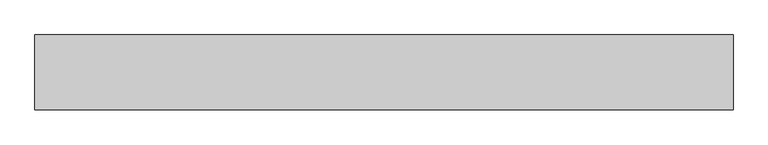
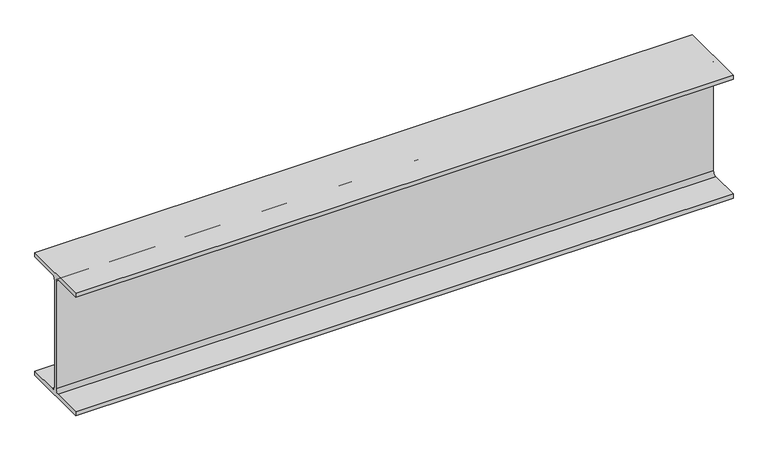
"""IFC4 building model written with IfcOpenShell, lengths in millimetres: beam geometry, Old_Steel Beam_H-KSD3502 : H_SB_ASB_H-194×150x6x9."""

from ifc_helpers import new_model, si_unit, point, frame, frame_2d, origin, place, context, project, spatial, polyline, circle_curve, trimmed, segment, composite_curve, outline, extrude, source, transform, mapped, element, save


def beam_1ed5de3b(model_context):
    return source(origin(), model_context, "Body", "SweptSolid", [
        extrude(outline(composite_curve([segment(polyline([(-82.5, -141.5), (-11.9, -141.5)]), True, "CONTINUOUS"), segment(trimmed(circle_curve(frame_2d((-11.9, -132.6)), 8.9), [point((-11.9, -141.5))], [point((-3.0, -132.6))], True, "CARTESIAN"), True, "CONTINUOUS"), segment(polyline([(-3.0, -132.6), (-3.0, 132.6)]), True, "CONTINUOUS"), segment(trimmed(circle_curve(frame_2d((-11.9, 132.6)), 8.9), [point((-3.0, 132.6))], [point((-11.9, 141.5))], True, "CARTESIAN"), True, "CONTINUOUS"), segment(polyline([(-11.9, 141.5), (-82.5, 141.5), (-82.5, 151.7), (82.5, 151.7), (82.5, 141.5), (11.9, 141.5)]), True, "CONTINUOUS"), segment(trimmed(circle_curve(frame_2d((11.9, 132.6)), 8.9), [point((11.9, 141.5))], [point((3.0, 132.6))], True, "CARTESIAN"), True, "CONTINUOUS"), segment(polyline([(3.0, 132.6), (3.0, -132.6)]), True, "CONTINUOUS"), segment(trimmed(circle_curve(frame_2d((11.9, -132.6)), 8.9), [point((3.0, -132.6))], [point((11.9, -141.5))], True, "CARTESIAN"), True, "CONTINUOUS"), segment(polyline([(11.9, -141.5), (82.5, -141.5), (82.5, -151.7), (-82.5, -151.7), (-82.5, -141.5)]), True, "CONTINUOUS")], self_intersect=False)), frame((-549.6452709, 0.0, 0.0), z_axis=(1.0, 0.0, 0.0), x_axis=(0.0, 1.0, 0.0)), (0.0, 0.0, 1.0), 1537.9998794),
    ])


if __name__ == "__main__":
    model = new_model("IFC4")
    model_context = context("Model", 3, world=origin())
    ifc_project = project(units=[si_unit("LENGTHUNIT", "METRE", prefix="MILLI")], contexts=[model_context])
    site = spatial("IfcSite", under=ifc_project)
    building = spatial("IfcBuilding", under=site)
    placement = place(None, origin())
    beam_shape = beam_1ed5de3b(model_context)
    element("IfcBeam", 1, ObjectType="Old_Steel Beam_H-KSD3502 : H_SB_ASB_H-194×150x6x9", at=placement, inside=building, context=model_context, shape_type="MappedRepresentation", body=[
        mapped(beam_shape, transform((0.0, 0.0, 0.0), x_axis=(1.0, 0.0, 0.0), y_axis=(0.0, 1.0, 0.0), z_axis=(0.0, 0.0, 1.0))),
    ])
    save(model, "model.ifc")

# Revit data of these elements
# Type "Old_Steel Beam_H-KSD3502 : H_SB_ASB_H-194×150x6x9"
#   Width = 15.0 cm
#   Web Thickness = 0.6 cm
#   Web Fillet = 1.3 cm
#   Warping Constant = 43316.0 cm⁶
#   Torsional Moment of Inertia = 8.622 cm⁴
#   Torsional Modulus = 1.0 cm³
#   Section Area = 39.01 cm²
#   Plastic Modulus weak axis = 104.0 cm³
#   Plastic Modulus strong axis = 309.0 cm³
#   Perimeter = 0.95 m²/m
#   Nominal Weight = 30.60 kgf/m
#   Moment of Inertia weak axis = 507.00 cm⁴
#   Moment of Inertia strong axis = 2690.00 cm⁴
#   Height = 19.4 cm
#   Flange Thickness = 0.9 cm
#   Elastic Modulus weak axis = 67.6 cm³
#   Elastic Modulus strong axis = 277.0 cm³
#   Centroid Vertical = 9.7 cm
#   Centroid Horizontal = 7.5 cm
#   Length [instance default] = 1.5240 m
#   Structural Material [instance default] = Steel, 45-345
#   Assembly Code = ""
# Element 1 (IfcBeam, "Old_Steel Beam_H-KSD3502 : H_SB_ASB_H-194×150x6x9")
#   Structural Material = none
# Materials
#   "Steel, 45-345": class "Metal", colour RGB 189 187 185, transparency 0, Description = "Steel 345 MPa", Cost = 0
